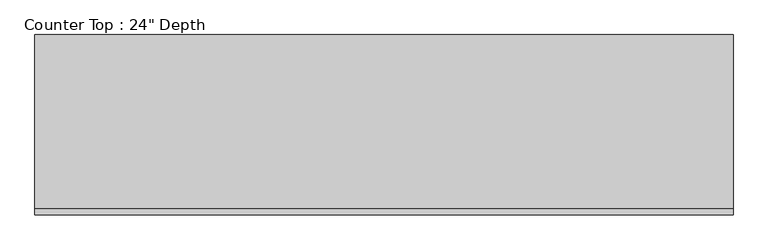
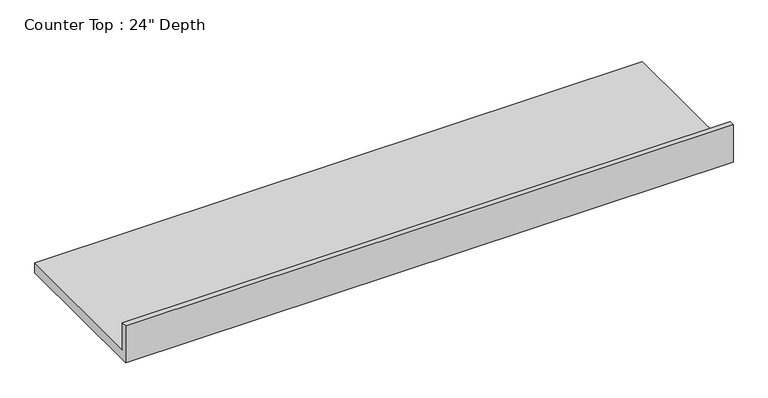
"""IFC4 building model written with IfcOpenShell, lengths in millimetres: furniture geometry."""

from ifc_helpers import new_model, si_unit, frame, origin, place, context, project, spatial, polyline, outline, extrude, source, transform, mapped, element, save


def furniture_bb1d5dfa(model_context):
    return source(origin(), model_context, "Body", "SweptSolid", [
        extrude(outline(polyline([(0.0, 1016.0), (19.05, 1016.0), (19.05, 914.4), (558.8, 914.4), (558.8, 876.3), (0.0, 876.3), (0.0, 1016.0)])), frame((-1200.4622951, 0.0, 0.0), z_axis=(1.0, 0.0, 0.0), x_axis=(0.0, 1.0, 0.0)), (0.0, 0.0, 1.0), 2162.175),
    ])


if __name__ == "__main__":
    model = new_model("IFC4")
    model_context = context("Model", 3, world=origin())
    ifc_project = project(units=[si_unit("LENGTHUNIT", "METRE", prefix="MILLI")], contexts=[model_context])
    site = spatial("IfcSite", under=ifc_project)
    building = spatial("IfcBuilding", under=site)
    placement = place(None, origin())
    furniture_shape = furniture_bb1d5dfa(model_context)
    element("IfcFurniture", 1, ObjectType="Counter Top : 24\" Depth", at=placement, inside=building, context=model_context, shape_type="MappedRepresentation", body=[
        mapped(furniture_shape, transform((0.0, 0.0, 0.0), x_axis=(1.0, 0.0, 0.0), y_axis=(0.0, 1.0, 0.0), z_axis=(0.0, 0.0, 1.0))),
    ])
    save(model, "model.ifc")

# Revit data of these elements
# Type "Counter Top : 24\" Depth"
#   Keynote = "M12366116.01"
#   Assembly Code = "C1030400"
#   Counter Thickness = 0' - 1 1/2"
#   Depth = 1' - 10"
#   Height = 3' - 0"
#   Length [instance default] = 8' - 0"
#   Counter Top Material = none
# Element 1 (IfcFurniture, "Counter Top : 24\" Depth")
#   Length = 7' - 1 1/8"
#   Materials on its faces: "CASEWORK"
# Materials
#   "CASEWORK": class "Generic", colour RGB 181 181 181, transparency 0, Cost = 0
